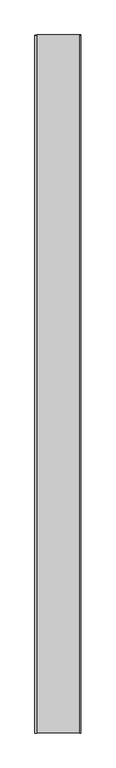
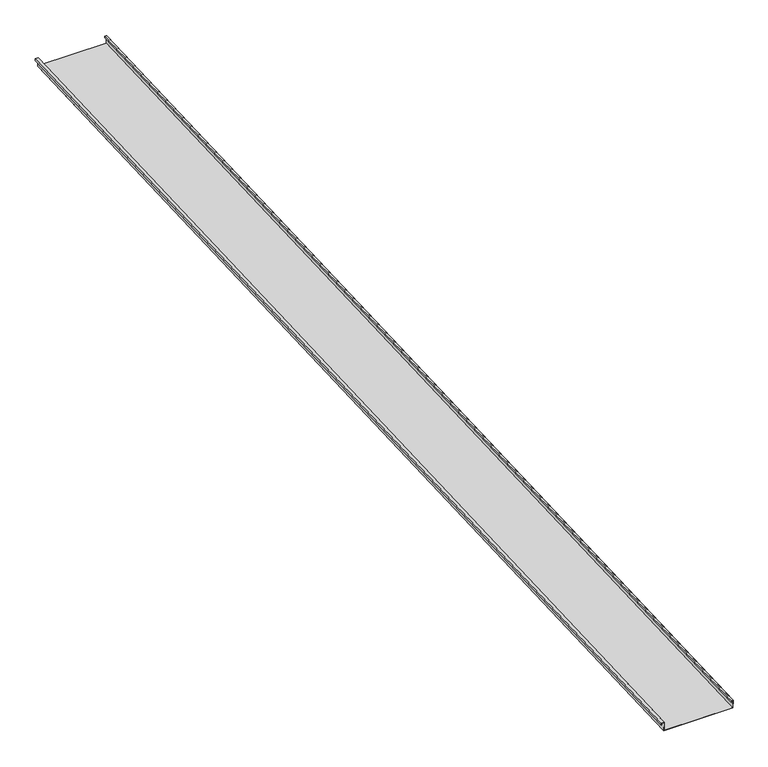
"""IFC4 building model written with IfcOpenShell, lengths in millimetres: proxy geometry, Generic Models 2:Generic Models 2:310765:Generic Models 2:310765 : Generic Models 2:Generic Models 2:310765:116 : Generic Models 2:Generic Models 2:310765:Generic Models 2:310765 : Generic Models 2:Generic Models 2:310765:300385."""

from ifc_helpers import new_model, si_unit, frame, origin, place, context, project, spatial, polyline, outline, extrude, source, transform, mapped, element, save


def generic_models_29faa235(model_context):
    return source(origin(), model_context, "Body", "SweptSolid", [
        extrude(outline(polyline([(1.5875, 0.0), (1.5875, 50.8), (407.9875, 50.8), (407.9875, 1.5875), (396.875, 1.5875), (396.875, 11.1125), (398.4625, 11.1125), (398.4625, 3.175), (406.4, 3.175), (406.4, 49.2125), (3.175, 49.2125), (3.175, -1.5874999), (-14.2875, -1.5874999), (-14.2875, 9.525), (-12.7, 9.525), (-12.7, 0.0), (1.5875, 0.0)])), frame((667069.2096405, -581354.4345603, 3902.6697972), z_axis=(0.0, 0.9991330730923568, 0.041630544712067834), x_axis=(1.0, 0.0, 0.0)), (0.0, 0.0, 1.0), 6400.8),
    ])


if __name__ == "__main__":
    model = new_model("IFC4")
    model_context = context("Model", 3, world=origin())
    ifc_project = project(units=[si_unit("LENGTHUNIT", "METRE", prefix="MILLI")], contexts=[model_context])
    site = spatial("IfcSite", under=ifc_project)
    building = spatial("IfcBuilding", under=site)
    placement = place(None, origin())
    generic_models_shape = generic_models_29faa235(model_context)
    element("IfcBuildingElementProxy", 1, Name="Generic Models 2:Generic Models 2:310765:Generic Models 2:310765 : Generic Models 2:Generic Models 2:310765:116 : Generic Models 2:Generic Models 2:310765:Generic Models 2:310765 : Generic Models 2:Generic Models 2:310765:300385", ObjectType="Generic Models 2:Generic Models 2:310765:Generic Models 2:310765 : Generic Models 2:Generic Models 2:310765:116 : Generic Models 2:Generic Models 2:310765:Generic Models 2:310765 : Generic Models 2:Generic Models 2:310765:300385", at=placement, inside=building, context=model_context, shape_type="MappedRepresentation", body=[
        mapped(generic_models_shape, transform((0.0, 0.0, 0.0), x_axis=(1.0, 0.0, 0.0), y_axis=(0.0, 1.0, 0.0), z_axis=(0.0, 0.0, 1.0))),
    ])
    save(model, "model.ifc")

# Revit data of these elements
# Type "Generic Models 2:Generic Models 2:310765:Generic Models 2:310765 : Generic Models 2:Generic Models 2:310765:116 : Generic Models 2:Generic Models 2:310765:Generic Models 2:310765 : Generic Models 2:Generic Models 2:310765:300385"
#   NameOverride = "Generic Models 2:Generic Models 2:310765:Generic Models 2:310765 : Generic Models 2:Generic Models 2:310765:300385"
#   ObjectTypeOverride = "Generic Models 2:310765 : Generic Models 2:Generic Models 2:310765"
#   Reference = "Generic Models 2"
#   Tag = "300385"
# Element 1 (IfcBuildingElementProxy, "Generic Models 2:Generic Models 2:310765:Generic Models 2:310765 : Generic Models 2:Generic Models 2:310765:116 : Generic Models 2:Generic Models 2:310765:Generic Models 2:310765 : Generic Models 2:Generic Models 2:310765:300385")
#   Materials on its faces: "THERMAL BROKEN ALUMINUM STOREFRONT FOR POLYCARBONATE"
# Materials
#   "THERMAL BROKEN ALUMINUM STOREFRONT FOR POLYCARBONATE": class "Unassigned", colour RGB 244 244 244, transparency 0, Keynote = "M07611300.01", Cost = 0
